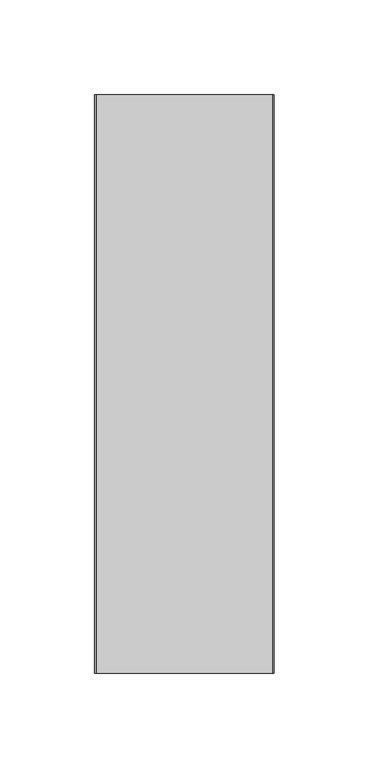
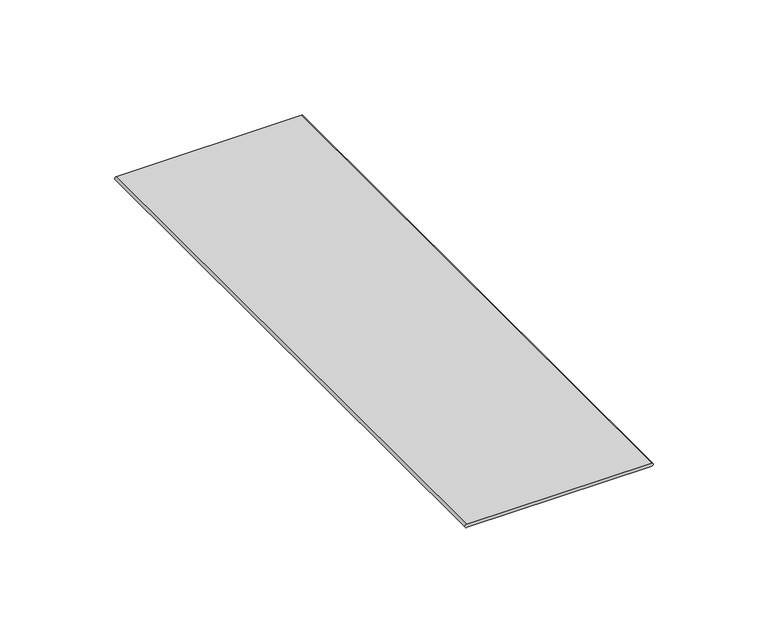
"""IFC4 building model written with IfcOpenShell, lengths in millimetres: proxy geometry, Generic Models 273:Generic Models 273:154836 : Generic Models 273:Generic Models 273:154836."""

import ifcopenshell
import ifcopenshell.guid

model = None  # the IFC model being written
_history = None  # IfcOwnerHistory: only IFC2X3 demands one
_inside = {}  # id of a spatial element -> (the spatial element, [elements in it])
_under = {}  # id of a project, library or spatial element -> (it, [spatial elements below it])
_declared = {}  # id of a project -> (the project, [libraries it declares])
_typed = {}  # id of a type object -> (the type object, [elements of that type])
_made_of = {}  # id of a material, layer set ... -> (it, [elements and type objects made of it])


def new_model(schema):
    """Start an empty IFC model of exactly this schema.

    Asked for "IFC4X3", IfcOpenShell would pick the latest addendum, in which some entities
    have other attributes; the version numbers below select the first issue.
    IFC2X3 requires an IfcOwnerHistory on every rooted entity: one is made here for all.
    """
    global model, _history
    if schema == "IFC4X3":
        model = ifcopenshell.file(schema_version=(4, 3, 0, 0))
    else:
        model = ifcopenshell.file(schema=schema)
    _inside.clear()
    _under.clear()
    _declared.clear()
    _typed.clear()
    _made_of.clear()
    _history = None
    if model.schema == "IFC2X3":
        org = make("IfcOrganization", Name="unknown")
        user = make(
            "IfcPersonAndOrganization",
            ThePerson=make("IfcPerson", FamilyName="unknown"),
            TheOrganization=org,
        )
        app = make(
            "IfcApplication",
            ApplicationDeveloper=org,
            Version="unknown",
            ApplicationFullName="unknown",
            ApplicationIdentifier="unknown",
        )
        _history = make(
            "IfcOwnerHistory",
            OwningUser=user,
            OwningApplication=app,
            ChangeAction="ADDED",
            CreationDate=0,
        )
    return model


def make(cls, **values):
    """One entity of the class cls with the attributes given. An attribute that is None is left unset."""
    return model.create_entity(
        cls, **{name: value for name, value in values.items() if value is not None}
    )


def rooted(cls, **values):
    """An entity with a GlobalId (a new one), such as an element, a storey or a relation."""
    return make(cls, GlobalId=ifcopenshell.guid.new(), OwnerHistory=_history, **values)


def si_unit(unit_type, name, prefix=None):
    """IfcSIUnit, for example si_unit("LENGTHUNIT", "METRE", prefix="MILLI")."""
    return make("IfcSIUnit", UnitType=unit_type, Prefix=prefix, Name=name)


def assignment(units):
    """IfcUnitAssignment: the units of a project."""
    return None if units is None else make("IfcUnitAssignment", Units=units)


def point(xyz):
    """IfcCartesianPoint."""
    return None if xyz is None else make("IfcCartesianPoint", Coordinates=xyz)


def direction(xyz):
    """IfcDirection."""
    return None if xyz is None else make("IfcDirection", DirectionRatios=xyz)


def frame(location, z_axis=None, x_axis=None):
    """IfcAxis2Placement3D, a coordinate frame: its origin and axes. An axis left out is left unset."""
    return make(
        "IfcAxis2Placement3D",
        Location=point(location),
        Axis=direction(z_axis),
        RefDirection=direction(x_axis),
    )


def frame_2d(location, x_axis=None):
    """IfcAxis2Placement2D, a coordinate frame in the plane: its origin and x axis."""
    return make(
        "IfcAxis2Placement2D", Location=point(location), RefDirection=direction(x_axis)
    )


def origin():
    """The frame at (0, 0, 0) with its axes left unset."""
    return frame((0.0, 0.0, 0.0))


def place(relative_to, where):
    """IfcLocalPlacement: puts the frame where relative to a parent placement (None: the world)."""
    return make(
        "IfcLocalPlacement", PlacementRelTo=relative_to, RelativePlacement=where
    )


def context(
    kind, dimensions, precision=None, world=None, true_north=None, identifier=None
):
    """IfcGeometricRepresentationContext, for example the 3D "Model" context."""
    return make(
        "IfcGeometricRepresentationContext",
        ContextIdentifier=identifier,
        ContextType=kind,
        CoordinateSpaceDimension=dimensions,
        Precision=precision,
        WorldCoordinateSystem=world,
        TrueNorth=true_north,
    )


def project(units=None, contexts=None):
    """IfcProject with its units and contexts."""
    return rooted(
        "IfcProject",
        Name="project",
        RepresentationContexts=contexts,
        UnitsInContext=assignment(units),
    )


def spatial(cls, under=None, at=None, **own):
    """A site, building, storey or space (cls), placed at a placement, below another one or the project."""
    s = rooted(cls, ObjectPlacement=at, **own)
    if under is not None:
        _under.setdefault(under.id(), (under, []))[1].append(s)
    return s


def polyline(points):
    """IfcPolyline through the points."""
    return make("IfcPolyline", Points=[point(p) for p in points])


def circle_curve(where, radius):
    """IfcCircle in the frame where."""
    return make("IfcCircle", Position=where, Radius=radius)


def trimmed(basis, trim1, trim2, sense, master):
    """IfcTrimmedCurve: the piece of a basis curve between two trims."""
    return make(
        "IfcTrimmedCurve",
        BasisCurve=basis,
        Trim1=trim1,
        Trim2=trim2,
        SenseAgreement=sense,
        MasterRepresentation=master,
    )


def segment(curve, same_sense, transition):
    """IfcCompositeCurveSegment."""
    return make(
        "IfcCompositeCurveSegment",
        Transition=transition,
        SameSense=same_sense,
        ParentCurve=curve,
    )


def composite_curve(segments, self_intersect=None):
    """IfcCompositeCurve: segments joined end to end."""
    return make("IfcCompositeCurve", Segments=segments, SelfIntersect=self_intersect)


def outline(outer, holes=None, kind="AREA"):
    """IfcArbitraryClosedProfileDef: a profile drawn as a closed curve; with holes, ...WithVoids."""
    if holes is None:
        return make("IfcArbitraryClosedProfileDef", ProfileType=kind, OuterCurve=outer)
    return make(
        "IfcArbitraryProfileDefWithVoids",
        ProfileType=kind,
        OuterCurve=outer,
        InnerCurves=holes,
    )


def extrude(swept, where, along, depth):
    """IfcExtrudedAreaSolid: the profile swept, set in the frame where, extruded along a direction by depth."""
    return make(
        "IfcExtrudedAreaSolid",
        SweptArea=swept,
        Position=where,
        ExtrudedDirection=direction(along),
        Depth=depth,
    )


def shape(context_of_items, identifier, shape_type, items):
    """IfcShapeRepresentation: the items that make up one representation, for example the "Body"."""
    return make(
        "IfcShapeRepresentation",
        ContextOfItems=context_of_items,
        RepresentationIdentifier=identifier,
        RepresentationType=shape_type,
        Items=items,
    )


def source(mapping_origin, context_of_items, identifier, shape_type, items):
    """IfcRepresentationMap: a shape defined once, which mapped items show again and again."""
    return make(
        "IfcRepresentationMap",
        MappingOrigin=mapping_origin,
        MappedRepresentation=shape(context_of_items, identifier, shape_type, items),
    )


def transform(
    local_origin,
    x_axis=None,
    y_axis=None,
    z_axis=None,
    scale=None,
    scale2=None,
    scale3=None,
    uniform=True,
):
    """IfcCartesianTransformationOperator3D, or its non-uniform kind. x_axis, y_axis, z_axis: its Axis1, 2, 3."""
    if uniform:
        return make(
            "IfcCartesianTransformationOperator3D",
            Axis1=direction(x_axis),
            Axis2=direction(y_axis),
            LocalOrigin=point(local_origin),
            Scale=scale,
            Axis3=direction(z_axis),
        )
    return make(
        "IfcCartesianTransformationOperator3DnonUniform",
        Axis1=direction(x_axis),
        Axis2=direction(y_axis),
        LocalOrigin=point(local_origin),
        Scale=scale,
        Axis3=direction(z_axis),
        Scale2=scale2,
        Scale3=scale3,
    )


def mapped(mapping_source, mapping_target):
    """IfcMappedItem: shows the shape of a source again, moved by a transform."""
    return make(
        "IfcMappedItem", MappingSource=mapping_source, MappingTarget=mapping_target
    )


def made_of(thing, what):
    """Note that an element or type object is made of a material, layer set ...; save() writes the relation."""
    if what is not None:
        _made_of.setdefault(what.id(), (what, []))[1].append(thing)
    return thing


def element(
    cls,
    number,
    at=None,
    inside=None,
    cuts=None,
    type_object=None,
    material=None,
    context=None,
    identifier="Body",
    shape_type=None,
    held_by="IfcProductDefinitionShape",
    body=None,
    shapes=None,
    **own,
):
    """One element of the class cls, such as IfcWall. Its Tag is "e" and its number.

    at: its placement. inside: the storey or other place that contains it. cuts: it is an
    opening in that element (IfcRelVoidsElement). A single representation is given by context,
    identifier, shape_type and body (its items); several are given by shapes. held_by: the class
    of the entity that holds the representations. save() writes the other relations.
    """
    e = rooted(cls, Tag="e%d" % number, ObjectPlacement=at, **own)
    if body is not None:
        shapes = [shape(context, identifier, shape_type, body)]
    if shapes is not None:
        e.Representation = make(held_by, Representations=shapes)
    if inside is not None:
        _inside.setdefault(inside.id(), (inside, []))[1].append(e)
    if cuts is not None:
        rooted(
            "IfcRelVoidsElement", RelatingBuildingElement=cuts, RelatedOpeningElement=e
        )
    if type_object is not None:
        _typed.setdefault(type_object.id(), (type_object, []))[1].append(e)
    return made_of(e, material)


def aggregate(whole, parts):
    """IfcRelAggregates: a whole, such as a stair, and the parts it consists of."""
    return rooted("IfcRelAggregates", RelatingObject=whole, RelatedObjects=parts)


def save(model, path):
    """Write the relations noted so far, then the file.

    IfcRelAggregates (storeys below a building ...), IfcRelContainedInSpatialStructure (elements
    in a storey), IfcRelDefinesByType, IfcRelAssociatesMaterial and IfcRelDeclares: one each for
    every whole, place, type object, material and project.
    """
    for whole, parts in _under.values():
        aggregate(whole, parts)
    for where, things in _inside.values():
        rooted(
            "IfcRelContainedInSpatialStructure",
            RelatedElements=things,
            RelatingStructure=where,
        )
    for kind, things in _typed.values():
        rooted("IfcRelDefinesByType", RelatedObjects=things, RelatingType=kind)
    for what, things in _made_of.values():
        rooted("IfcRelAssociatesMaterial", RelatedObjects=things, RelatingMaterial=what)
    for by, libraries in _declared.values():
        rooted("IfcRelDeclares", RelatingContext=by, RelatedDefinitions=libraries)
    model.write(path)


def generic_models_7ca5872b(model_context):
    return source(origin(), model_context, "Body", "SweptSolid", [
        extrude(outline(composite_curve([segment(polyline([(139.4429787, 1483.7900601), (139.4429787, 1576.7947677)]), True, "CONTINUOUS"), segment(trimmed(circle_curve(frame_2d((140.2367287, 1576.7947677)), 0.79375), [point((139.4429787, 1576.7947677))], [point((141.0304787, 1576.7947677))], False, "CARTESIAN"), True, "CONTINUOUS"), segment(polyline([(141.0304787, 1576.7947677), (141.0304787, 1483.7900601)]), True, "CONTINUOUS"), segment(trimmed(circle_curve(frame_2d((140.2367287, 1483.7900601)), 0.79375), [point((141.0304787, 1483.7900601))], [point((139.4429787, 1483.7900601))], False, "CARTESIAN"), True, "CONTINUOUS")], self_intersect=False)), frame((0.0, 4450.212823, 0.0), z_axis=(0.0, 1.0, 0.0), x_axis=(0.0, 0.0, 1.0)), (0.0, 0.0, 1.0), 304.8),
    ])


if __name__ == "__main__":
    model = new_model("IFC4")
    model_context = context("Model", 3, world=origin())
    ifc_project = project(units=[si_unit("LENGTHUNIT", "METRE", prefix="MILLI")], contexts=[model_context])
    site = spatial("IfcSite", under=ifc_project)
    building = spatial("IfcBuilding", under=site)
    placement = place(None, origin())
    generic_models_shape = generic_models_7ca5872b(model_context)
    element("IfcBuildingElementProxy", 1, Name="Generic Models 273:Generic Models 273:154836 : Generic Models 273:Generic Models 273:154836", ObjectType="Generic Models 273:Generic Models 273:154836 : Generic Models 273:Generic Models 273:154836", at=placement, inside=building, context=model_context, shape_type="MappedRepresentation", body=[
        mapped(generic_models_shape, transform((0.0, 0.0, 0.0), x_axis=(1.0, 0.0, 0.0), y_axis=(0.0, 1.0, 0.0), z_axis=(0.0, 0.0, 1.0))),
    ])
    save(model, "model.ifc")

# Revit data of these elements
# Type "Generic Models 273:Generic Models 273:154836 : Generic Models 273:Generic Models 273:154836"
#   NameOverride = "Generic Models 273:Generic Models 273:154836"
#   ObjectTypeOverride = "Generic Models 273:Generic Models 273"
#   Reference = "Generic Models 273"
#   Category = "Generic Models"
#   Tag = "154836"
# Element 1 (IfcBuildingElementProxy, "Generic Models 273:Generic Models 273:154836 : Generic Models 273:Generic Models 273:154836")
#   Materials on its faces: "_BED OF SEALANT 27222"
# Materials
#   "_BED OF SEALANT 27222": class "Unassigned", colour RGB 253 192 103, transparency 0
